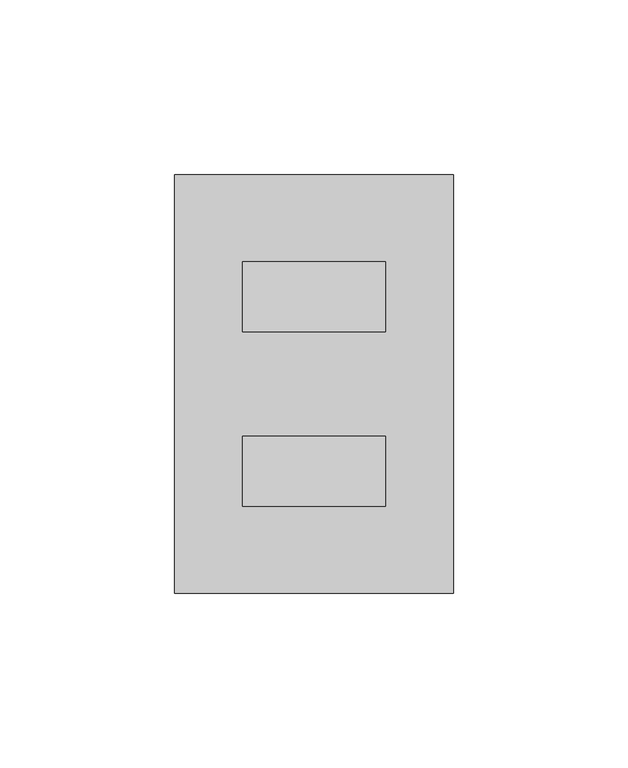
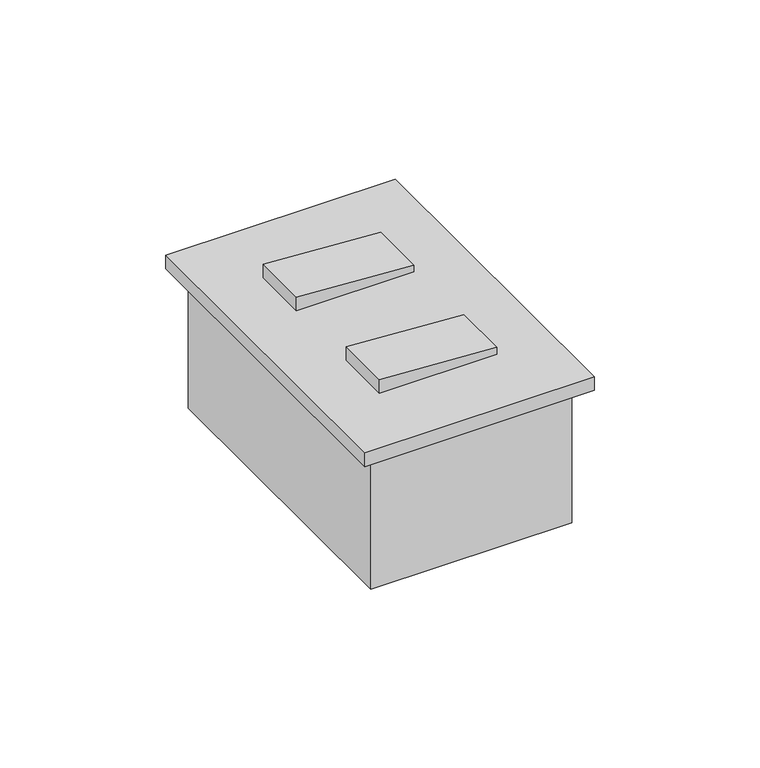
"""IFC4 building model written with IfcOpenShell, lengths in millimetres: proxy geometry, CAIXA VERTICE V7 : Interruptor 2s."""

from ifc_helpers import new_model, si_unit, frame, origin, origin_with_axes, place, context, project, spatial, polyline, outline, extrude, faceted_brep, source, transform, mapped, element, save


def electrical_fixtures_175ece23(model_context):
    return source(origin(), model_context, "Body", "SolidModel", [
        extrude(outline(polyline([(5.0, 20.5), (7.5, 20.5), (10.0, -20.5), (5.0, -20.5), (5.0, 20.5)])), frame((0.0, -1085.0, 0.0), z_axis=(0.0, 1.0, 0.0), x_axis=(0.0, 0.0, 1.0)), (0.0, 0.0, 1.0), 20.0),
        extrude(outline(polyline([(5.0, 20.5), (7.5, 20.5), (10.0, -20.5), (5.0, -20.5), (5.0, 20.5)])), frame((0.0, -1135.0, 0.0), z_axis=(0.0, 1.0, 0.0), x_axis=(0.0, 0.0, 1.0)), (0.0, 0.0, 1.0), 20.0),
        faceted_brep([(35.0, -1155.0, 0.0), (35.0, -1045.0, 0.0), (-35.0, -1045.0, 0.0), (-35.0, -1155.0, 0.0), (33.0, -1153.0, 0.0), (-33.0, -1153.0, 0.0), (-33.0, -1047.0, 0.0), (33.0, -1047.0, 0.0), (33.0, -1047.0, -48.0), (-33.0, -1047.0, -48.0), (-33.0, -1153.0, -48.0), (33.0, -1153.0, -48.0), (35.0, -1155.0, -50.0), (-35.0, -1155.0, -50.0), (-35.0, -1045.0, -50.0), (35.0, -1045.0, -50.0)], [[[0, 1, 2, 3], [4, 5, 6, 7]], [[8, 9, 10, 11]], [[12, 13, 14, 15]], [[12, 0, 3, 13]], [[3, 2, 14, 13]], [[2, 1, 15, 14]], [[1, 0, 12, 15]], [[7, 8, 11, 4]], [[6, 9, 8, 7]], [[5, 10, 9, 6]], [[4, 11, 10, 5]]]),
        extrude(outline(polyline([(40.0, -1160.0), (-40.0, -1160.0), (-40.0, -1040.0), (40.0, -1040.0), (40.0, -1160.0)])), origin_with_axes(), (0.0, 0.0, 1.0), 5.0),
    ])


if __name__ == "__main__":
    model = new_model("IFC4")
    model_context = context("Model", 3, world=origin())
    ifc_project = project(units=[si_unit("LENGTHUNIT", "METRE", prefix="MILLI")], contexts=[model_context])
    site = spatial("IfcSite", under=ifc_project)
    building = spatial("IfcBuilding", under=site)
    placement = place(None, origin())
    electrical_fixtures_shape = electrical_fixtures_175ece23(model_context)
    element("IfcBuildingElementProxy", 1, Name="CAIXA VERTICE V7 : Interruptor 2s", ObjectType="CAIXA VERTICE V7 : Interruptor 2s", at=placement, inside=building, context=model_context, shape_type="MappedRepresentation", body=[
        mapped(electrical_fixtures_shape, transform((0.0, 0.0, 0.0), x_axis=(1.0, 0.0, 0.0), y_axis=(0.0, 1.0, 0.0), z_axis=(0.0, 0.0, 1.0))),
    ])
    save(model, "model.ifc")

# Revit data of these elements
# Type "CAIXA VERTICE V7 : Interruptor 2s"
#   URL = "www.facebook.com/verticetreinamentos"
#   SEÇÃO [instance default] = ""
#   Rotação [instance default] = 0.00°
#   LARGURA DA TAMPA = 0.08 m
#   BORDA = 0.01 m
#   ALTURA DE INSTALAÇÃO [instance default] = 1.10 m
#   Distância Anotação [instance default] = 0.0015 m
#   ALTURA DA TAMPA = 0.12 m
#   Vertical [instance default] = yes
#   VER SEÇÃO [instance default] = yes
#   SHADE ESQ [instance default] = no
#   SHADE DIR [instance default] = yes
#   HORIZONTAL [instance default] = no
#   ANDAR COM A LEGENDA [instance default] = 0
#   Material Tampa [instance default] = Plástico, branco opaco
#   Caixa = element 1798510
#   Anotação = element 1798523
#   Default Elevation = 0
# Element 1 (IfcBuildingElementProxy, "CAIXA VERTICE V7 : Interruptor 2s")
#   SEÇÃO = "2"
#   Distância Anotação = 0.0055 m
#   ANDAR COM A LEGENDA = 2
#   Materials on its faces: "Plástico, branco opaco"
# Materials
#   "Plástico, branco opaco": class "Plástico", colour RGB 120 120 120, transparency 0, Description = "Plastic, generic, opaque white", Cost = 0
